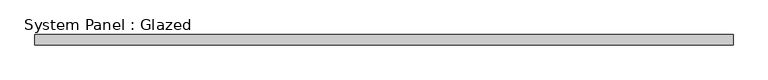
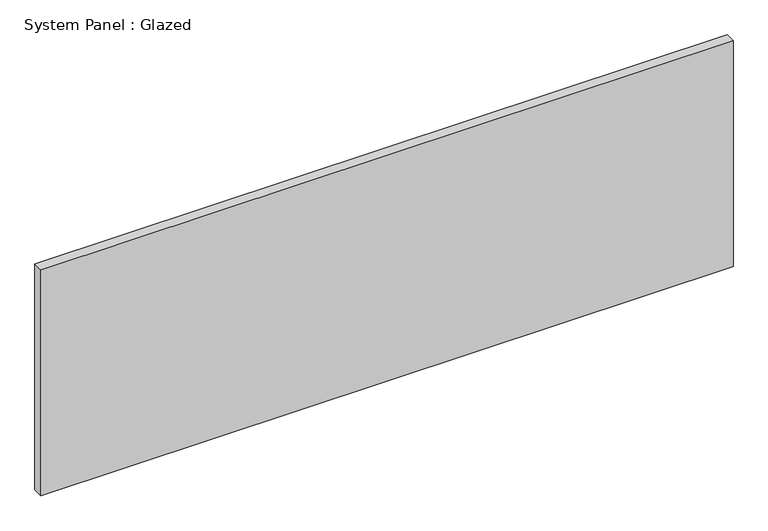
"""IFC4 building model written with IfcOpenShell, lengths in millimetres: plate geometry, System Panel : Glazed."""

from ifc_helpers import new_model, si_unit, origin, origin_with_axes, place, context, project, spatial, polyline, outline, extrude, source, transform, mapped, element, save


def system_panel_glazed_898e2a00(model_context):
    return source(origin(), model_context, "Body", "SweptSolid", [
        extrude(outline(polyline([(832.5, 24.5), (-832.5, 24.5), (-832.5, 49.5), (832.5, 49.5), (832.5, 24.5)])), origin_with_axes(), (0.0, 0.0, 1.0), 575.0),
    ])


if __name__ == "__main__":
    model = new_model("IFC4")
    model_context = context("Model", 3, world=origin())
    ifc_project = project(units=[si_unit("LENGTHUNIT", "METRE", prefix="MILLI")], contexts=[model_context])
    site = spatial("IfcSite", under=ifc_project)
    building = spatial("IfcBuilding", under=site)
    placement = place(None, origin())
    system_panel_glazed_shape = system_panel_glazed_898e2a00(model_context)
    element("IfcPlate", 1, ObjectType="System Panel : Glazed", at=placement, inside=building, context=model_context, shape_type="MappedRepresentation", body=[
        mapped(system_panel_glazed_shape, transform((0.0, 0.0, 0.0), x_axis=(1.0, 0.0, 0.0), y_axis=(0.0, 1.0, 0.0), z_axis=(0.0, 0.0, 1.0))),
    ])
    save(model, "model.ifc")

# Revit data of these elements
# Element 1 (IfcPlate, "System Panel : Glazed")
#   Materials on its faces: "Glass"
# Materials
#   "Glass": class "Glass", colour RGB 218 227 224, transparency 0.85, Description = "Soda Lime Glass", Cost = 0
